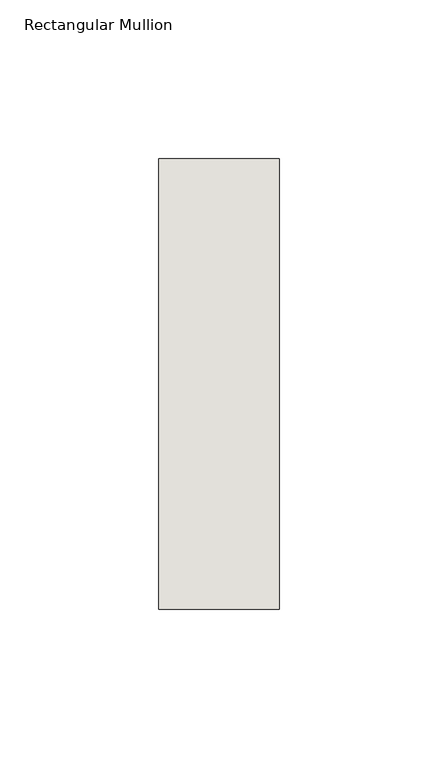
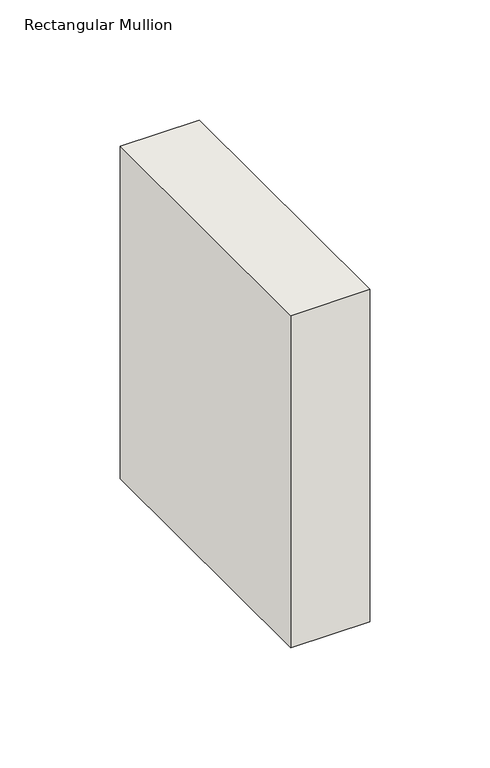
"""IFC4 building model written with IfcOpenShell, lengths in millimetres: wall geometry, Rectangular Mullion : NLRS_21_CWM_hsb-regel 38x142_gen_rsf."""

from ifc_helpers import new_model, si_unit, frame, origin, place, context, project, spatial, polyline, outline, extrude, source, transform, mapped, element, save


def rectangular_mullion_1f17af45(model_context):
    return source(origin(), model_context, "Body", "SweptSolid", [
        extrude(outline(polyline([(0.0, -71.0), (-38.0, -71.0), (-38.0, 71.0), (0.0, 71.0), (0.0, -71.0)])), frame((0.0, 0.0, -168.9999997), z_axis=(0.0, 0.0, 1.0), x_axis=(1.0, 0.0, 0.0)), (0.0, 0.0, 1.0), 168.9999997),
    ])


if __name__ == "__main__":
    model = new_model("IFC4")
    model_context = context("Model", 3, world=origin())
    ifc_project = project(units=[si_unit("LENGTHUNIT", "METRE", prefix="MILLI")], contexts=[model_context])
    site = spatial("IfcSite", under=ifc_project)
    building = spatial("IfcBuilding", under=site)
    placement = place(None, origin())
    rectangular_mullion_shape = rectangular_mullion_1f17af45(model_context)
    element("IfcWall", 1, ObjectType="Rectangular Mullion : NLRS_21_CWM_hsb-regel 38x142_gen_rsf", at=placement, inside=building, context=model_context, shape_type="MappedRepresentation", body=[
        mapped(rectangular_mullion_shape, transform((0.0, 0.0, 0.0), x_axis=(1.0, 0.0, 0.0), y_axis=(0.0, 1.0, 0.0), z_axis=(0.0, 0.0, 1.0))),
    ])
    save(model, "model.ifc")

# Revit data of these elements
# Type "Rectangular Mullion : NLRS_21_CWM_hsb-regel 38x142_gen_rsf"
#   Type IfcGUID = "07M7mRoiH1CR8m_RSKIwpF"
#   Assembly Code = "21.10"
#   IfcExportAs = "IfcWall"
#   built-in parameter 1007322 = 0.465879 (stored number, unit not read)
#   built-in parameter 1007321 = 0.062336 (stored number, unit not read)
#   built-in parameter 1007320 = 0.062336 (stored number, unit not read)
# Element 1 (IfcWall, "Rectangular Mullion : NLRS_21_CWM_hsb-regel 38x142_gen_rsf")
#   Materials on its faces: "NLRS_i2_hout naaldhout vuren_gen_rsf"
# Materials
#   "NLRS_i2_hout naaldhout vuren_gen_rsf": class "I - Hout", colour RGB 234 199 147, transparency 0, Keynote = "i2", Manufacturer = "Revit Standards Foundation", URL = "www.revitstandards.org", Description = "hout vuren", Cost = 0
